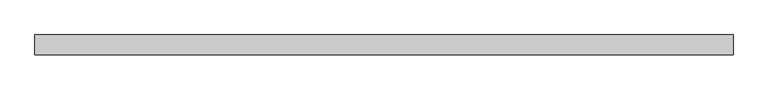
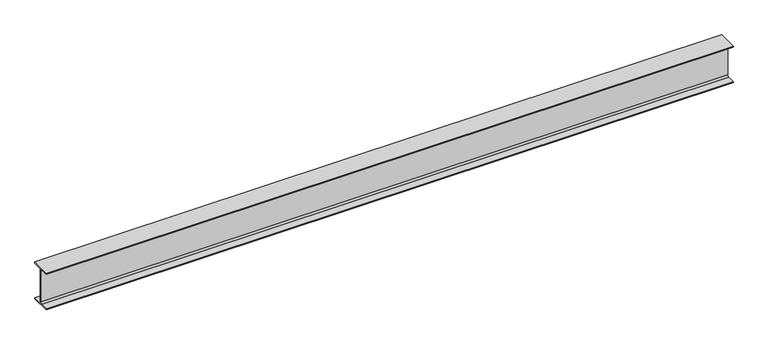
"""IFC4 building model written with IfcOpenShell, lengths in millimetres: beam geometry, 0912_Steel Framing_H-KSD3502 : H_SB_ASB_H-350x175x7x11."""

import ifcopenshell
import ifcopenshell.guid

model = None  # the IFC model being written
_history = None  # IfcOwnerHistory: only IFC2X3 demands one
_inside = {}  # id of a spatial element -> (the spatial element, [elements in it])
_under = {}  # id of a project, library or spatial element -> (it, [spatial elements below it])
_declared = {}  # id of a project -> (the project, [libraries it declares])
_typed = {}  # id of a type object -> (the type object, [elements of that type])
_made_of = {}  # id of a material, layer set ... -> (it, [elements and type objects made of it])


def new_model(schema):
    """Start an empty IFC model of exactly this schema.

    Asked for "IFC4X3", IfcOpenShell would pick the latest addendum, in which some entities
    have other attributes; the version numbers below select the first issue.
    IFC2X3 requires an IfcOwnerHistory on every rooted entity: one is made here for all.
    """
    global model, _history
    if schema == "IFC4X3":
        model = ifcopenshell.file(schema_version=(4, 3, 0, 0))
    else:
        model = ifcopenshell.file(schema=schema)
    _inside.clear()
    _under.clear()
    _declared.clear()
    _typed.clear()
    _made_of.clear()
    _history = None
    if model.schema == "IFC2X3":
        org = make("IfcOrganization", Name="unknown")
        user = make(
            "IfcPersonAndOrganization",
            ThePerson=make("IfcPerson", FamilyName="unknown"),
            TheOrganization=org,
        )
        app = make(
            "IfcApplication",
            ApplicationDeveloper=org,
            Version="unknown",
            ApplicationFullName="unknown",
            ApplicationIdentifier="unknown",
        )
        _history = make(
            "IfcOwnerHistory",
            OwningUser=user,
            OwningApplication=app,
            ChangeAction="ADDED",
            CreationDate=0,
        )
    return model


def make(cls, **values):
    """One entity of the class cls with the attributes given. An attribute that is None is left unset."""
    return model.create_entity(
        cls, **{name: value for name, value in values.items() if value is not None}
    )


def rooted(cls, **values):
    """An entity with a GlobalId (a new one), such as an element, a storey or a relation."""
    return make(cls, GlobalId=ifcopenshell.guid.new(), OwnerHistory=_history, **values)


def si_unit(unit_type, name, prefix=None):
    """IfcSIUnit, for example si_unit("LENGTHUNIT", "METRE", prefix="MILLI")."""
    return make("IfcSIUnit", UnitType=unit_type, Prefix=prefix, Name=name)


def assignment(units):
    """IfcUnitAssignment: the units of a project."""
    return None if units is None else make("IfcUnitAssignment", Units=units)


def point(xyz):
    """IfcCartesianPoint."""
    return None if xyz is None else make("IfcCartesianPoint", Coordinates=xyz)


def direction(xyz):
    """IfcDirection."""
    return None if xyz is None else make("IfcDirection", DirectionRatios=xyz)


def frame(location, z_axis=None, x_axis=None):
    """IfcAxis2Placement3D, a coordinate frame: its origin and axes. An axis left out is left unset."""
    return make(
        "IfcAxis2Placement3D",
        Location=point(location),
        Axis=direction(z_axis),
        RefDirection=direction(x_axis),
    )


def frame_2d(location, x_axis=None):
    """IfcAxis2Placement2D, a coordinate frame in the plane: its origin and x axis."""
    return make(
        "IfcAxis2Placement2D", Location=point(location), RefDirection=direction(x_axis)
    )


def origin():
    """The frame at (0, 0, 0) with its axes left unset."""
    return frame((0.0, 0.0, 0.0))


def place(relative_to, where):
    """IfcLocalPlacement: puts the frame where relative to a parent placement (None: the world)."""
    return make(
        "IfcLocalPlacement", PlacementRelTo=relative_to, RelativePlacement=where
    )


def context(
    kind, dimensions, precision=None, world=None, true_north=None, identifier=None
):
    """IfcGeometricRepresentationContext, for example the 3D "Model" context."""
    return make(
        "IfcGeometricRepresentationContext",
        ContextIdentifier=identifier,
        ContextType=kind,
        CoordinateSpaceDimension=dimensions,
        Precision=precision,
        WorldCoordinateSystem=world,
        TrueNorth=true_north,
    )


def project(units=None, contexts=None):
    """IfcProject with its units and contexts."""
    return rooted(
        "IfcProject",
        Name="project",
        RepresentationContexts=contexts,
        UnitsInContext=assignment(units),
    )


def spatial(cls, under=None, at=None, **own):
    """A site, building, storey or space (cls), placed at a placement, below another one or the project."""
    s = rooted(cls, ObjectPlacement=at, **own)
    if under is not None:
        _under.setdefault(under.id(), (under, []))[1].append(s)
    return s


def polyline(points):
    """IfcPolyline through the points."""
    return make("IfcPolyline", Points=[point(p) for p in points])


def circle_curve(where, radius):
    """IfcCircle in the frame where."""
    return make("IfcCircle", Position=where, Radius=radius)


def trimmed(basis, trim1, trim2, sense, master):
    """IfcTrimmedCurve: the piece of a basis curve between two trims."""
    return make(
        "IfcTrimmedCurve",
        BasisCurve=basis,
        Trim1=trim1,
        Trim2=trim2,
        SenseAgreement=sense,
        MasterRepresentation=master,
    )


def segment(curve, same_sense, transition):
    """IfcCompositeCurveSegment."""
    return make(
        "IfcCompositeCurveSegment",
        Transition=transition,
        SameSense=same_sense,
        ParentCurve=curve,
    )


def composite_curve(segments, self_intersect=None):
    """IfcCompositeCurve: segments joined end to end."""
    return make("IfcCompositeCurve", Segments=segments, SelfIntersect=self_intersect)


def outline(outer, holes=None, kind="AREA"):
    """IfcArbitraryClosedProfileDef: a profile drawn as a closed curve; with holes, ...WithVoids."""
    if holes is None:
        return make("IfcArbitraryClosedProfileDef", ProfileType=kind, OuterCurve=outer)
    return make(
        "IfcArbitraryProfileDefWithVoids",
        ProfileType=kind,
        OuterCurve=outer,
        InnerCurves=holes,
    )


def extrude(swept, where, along, depth):
    """IfcExtrudedAreaSolid: the profile swept, set in the frame where, extruded along a direction by depth."""
    return make(
        "IfcExtrudedAreaSolid",
        SweptArea=swept,
        Position=where,
        ExtrudedDirection=direction(along),
        Depth=depth,
    )


def shape(context_of_items, identifier, shape_type, items):
    """IfcShapeRepresentation: the items that make up one representation, for example the "Body"."""
    return make(
        "IfcShapeRepresentation",
        ContextOfItems=context_of_items,
        RepresentationIdentifier=identifier,
        RepresentationType=shape_type,
        Items=items,
    )


def source(mapping_origin, context_of_items, identifier, shape_type, items):
    """IfcRepresentationMap: a shape defined once, which mapped items show again and again."""
    return make(
        "IfcRepresentationMap",
        MappingOrigin=mapping_origin,
        MappedRepresentation=shape(context_of_items, identifier, shape_type, items),
    )


def transform(
    local_origin,
    x_axis=None,
    y_axis=None,
    z_axis=None,
    scale=None,
    scale2=None,
    scale3=None,
    uniform=True,
):
    """IfcCartesianTransformationOperator3D, or its non-uniform kind. x_axis, y_axis, z_axis: its Axis1, 2, 3."""
    if uniform:
        return make(
            "IfcCartesianTransformationOperator3D",
            Axis1=direction(x_axis),
            Axis2=direction(y_axis),
            LocalOrigin=point(local_origin),
            Scale=scale,
            Axis3=direction(z_axis),
        )
    return make(
        "IfcCartesianTransformationOperator3DnonUniform",
        Axis1=direction(x_axis),
        Axis2=direction(y_axis),
        LocalOrigin=point(local_origin),
        Scale=scale,
        Axis3=direction(z_axis),
        Scale2=scale2,
        Scale3=scale3,
    )


def mapped(mapping_source, mapping_target):
    """IfcMappedItem: shows the shape of a source again, moved by a transform."""
    return make(
        "IfcMappedItem", MappingSource=mapping_source, MappingTarget=mapping_target
    )


def made_of(thing, what):
    """Note that an element or type object is made of a material, layer set ...; save() writes the relation."""
    if what is not None:
        _made_of.setdefault(what.id(), (what, []))[1].append(thing)
    return thing


def element(
    cls,
    number,
    at=None,
    inside=None,
    cuts=None,
    type_object=None,
    material=None,
    context=None,
    identifier="Body",
    shape_type=None,
    held_by="IfcProductDefinitionShape",
    body=None,
    shapes=None,
    **own,
):
    """One element of the class cls, such as IfcWall. Its Tag is "e" and its number.

    at: its placement. inside: the storey or other place that contains it. cuts: it is an
    opening in that element (IfcRelVoidsElement). A single representation is given by context,
    identifier, shape_type and body (its items); several are given by shapes. held_by: the class
    of the entity that holds the representations. save() writes the other relations.
    """
    e = rooted(cls, Tag="e%d" % number, ObjectPlacement=at, **own)
    if body is not None:
        shapes = [shape(context, identifier, shape_type, body)]
    if shapes is not None:
        e.Representation = make(held_by, Representations=shapes)
    if inside is not None:
        _inside.setdefault(inside.id(), (inside, []))[1].append(e)
    if cuts is not None:
        rooted(
            "IfcRelVoidsElement", RelatingBuildingElement=cuts, RelatedOpeningElement=e
        )
    if type_object is not None:
        _typed.setdefault(type_object.id(), (type_object, []))[1].append(e)
    return made_of(e, material)


def aggregate(whole, parts):
    """IfcRelAggregates: a whole, such as a stair, and the parts it consists of."""
    return rooted("IfcRelAggregates", RelatingObject=whole, RelatedObjects=parts)


def save(model, path):
    """Write the relations noted so far, then the file.

    IfcRelAggregates (storeys below a building ...), IfcRelContainedInSpatialStructure (elements
    in a storey), IfcRelDefinesByType, IfcRelAssociatesMaterial and IfcRelDeclares: one each for
    every whole, place, type object, material and project.
    """
    for whole, parts in _under.values():
        aggregate(whole, parts)
    for where, things in _inside.values():
        rooted(
            "IfcRelContainedInSpatialStructure",
            RelatedElements=things,
            RelatingStructure=where,
        )
    for kind, things in _typed.values():
        rooted("IfcRelDefinesByType", RelatedObjects=things, RelatingType=kind)
    for what, things in _made_of.values():
        rooted("IfcRelAssociatesMaterial", RelatedObjects=things, RelatingMaterial=what)
    for by, libraries in _declared.values():
        rooted("IfcRelDeclares", RelatingContext=by, RelatedDefinitions=libraries)
    model.write(path)


def beam_a4f2fb3b(model_context):
    return source(origin(), model_context, "Body", "SweptSolid", [
        extrude(outline(composite_curve([segment(polyline([(87.5, -164.0), (87.5, -175.0), (-87.5, -175.0), (-87.5, -164.0), (-17.5, -164.0)]), True, "CONTINUOUS"), segment(trimmed(circle_curve(frame_2d((-17.5, -150.0)), 14.0), [point((-17.5, -164.0))], [point((-3.5, -150.0))], True, "CARTESIAN"), True, "CONTINUOUS"), segment(polyline([(-3.5, -150.0), (-3.5, 150.0)]), True, "CONTINUOUS"), segment(trimmed(circle_curve(frame_2d((-17.5, 150.0)), 14.0), [point((-3.5, 150.0))], [point((-17.5, 164.0))], True, "CARTESIAN"), True, "CONTINUOUS"), segment(polyline([(-17.5, 164.0), (-87.5, 164.0), (-87.5, 175.0), (87.5, 175.0), (87.5, 164.0), (17.5, 164.0)]), True, "CONTINUOUS"), segment(trimmed(circle_curve(frame_2d((17.5, 150.0)), 14.0), [point((17.5, 164.0))], [point((3.5, 150.0))], True, "CARTESIAN"), True, "CONTINUOUS"), segment(polyline([(3.5, 150.0), (3.5, -150.0)]), True, "CONTINUOUS"), segment(trimmed(circle_curve(frame_2d((17.5, -150.0)), 14.0), [point((3.5, -150.0))], [point((17.5, -164.0))], True, "CARTESIAN"), True, "CONTINUOUS"), segment(polyline([(17.5, -164.0), (87.5, -164.0)]), True, "CONTINUOUS")], self_intersect=False)), frame((-3087.3, 0.0, 0.0), z_axis=(1.0, 0.0, 0.0), x_axis=(0.0, 1.0, 0.0)), (0.0, 0.0, 1.0), 6174.6),
    ])


if __name__ == "__main__":
    model = new_model("IFC4")
    model_context = context("Model", 3, world=origin())
    ifc_project = project(units=[si_unit("LENGTHUNIT", "METRE", prefix="MILLI")], contexts=[model_context])
    site = spatial("IfcSite", under=ifc_project)
    building = spatial("IfcBuilding", under=site)
    placement = place(None, origin())
    beam_shape = beam_a4f2fb3b(model_context)
    element("IfcBeam", 1, ObjectType="0912_Steel Framing_H-KSD3502 : H_SB_ASB_H-350x175x7x11", at=placement, inside=building, context=model_context, shape_type="MappedRepresentation", body=[
        mapped(beam_shape, transform((0.0, 0.0, 0.0), x_axis=(1.0, 0.0, 0.0), y_axis=(0.0, 1.0, 0.0), z_axis=(0.0, 0.0, 1.0))),
    ])
    save(model, "model.ifc")

# Revit data of these elements
# Type "0912_Steel Framing_H-KSD3502 : H_SB_ASB_H-350x175x7x11"
#   H_WM Code_1 = "S01AA002-00001 | Main Steel Structure Fabrication Work | Shelter/Building | Medium Steel - Standard (90KG/M>Weight≥30KG/M) | Material: (   )"
#   H_WM Code_2 = "S03AA028-00001 | Main Steel Structure Erection Work | Shelter/Building | Medium Steel (90KG/M>Weight≥30KG/M) | Material: (   )"
#   H_WM Code_3 = "S01AA010-00001 | Main Steel Structure Fabrication Work | Shelter/Building | Steel Painting/Coating | for Non-Fireproofed Steel Surface, Surface Preparation, Primer, Second & Final Coat | Material: (   )"
#   H_Q'ty Cal Type Tag = "SB-Q2"
#   Width = 17.5 cm
#   Web Thickness = 0.7 cm
#   Web Fillet = 1.4 cm
#   Warping Constant = 282000.0 cm⁶
#   W = 0
#   Torsional Moment of Inertia = 19.4042 cm⁴
#   Section Area = 63.14 cm²
#   Plastic Modulus weak axis = 174.0 cm³
#   Plastic Modulus strong axis = 868.0 cm³
#   Perimeter = 1.36 m²/m
#   Nominal Weight = 49.60 kgf/m
#   Moment of Inertia weak axis = 984.00 cm⁴
#   Moment of Inertia strong axis = 13600.00 cm⁴
#   Height = 35.0 cm
#   Flange Thickness = 1.1 cm
#   Elastic Modulus weak axis = 112.0 cm³
#   Elastic Modulus strong axis = 775.0 cm³
#   Centroid Vertical = 17.5 cm
#   Centroid Horizontal = 8.75 cm
#   Ix = 136000000
#   Length [instance default] = 1.5240 m
#   Zx = 868000
#   b = 0.1750 m
#   h = 0.3500 m
#   r = 0.0140 m
#   s = 0.0070 m
#   t = 0.0110 m
#   A = 0.006314 m²
#   Structural Material [instance default] = Steel, 45-345
#   Assembly Code = ""
# Element 1 (IfcBeam, "0912_Steel Framing_H-KSD3502 : H_SB_ASB_H-350x175x7x11")
#   Structural Material = none
# Materials
#   "Steel, 45-345": class "Metal", colour RGB 189 187 185, transparency 0, Description = "Steel 345 MPa", Cost = 0
